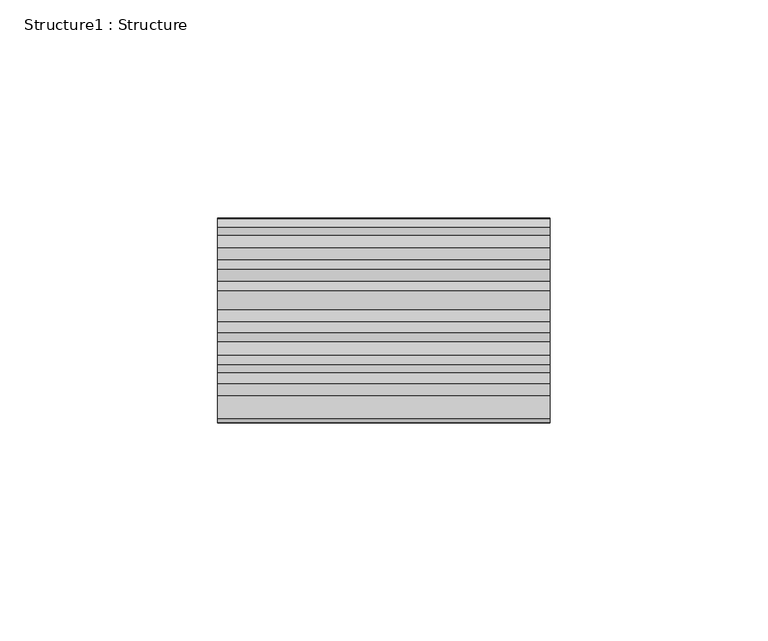
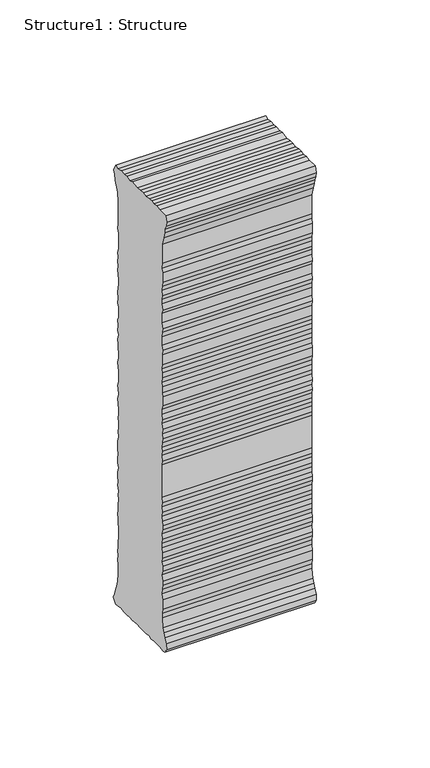
"""IFC4 building model written with IfcOpenShell, lengths in millimetres: proxy geometry, Structure1 : Structure."""

from ifc_helpers import new_model, si_unit, frame, origin, place, context, project, spatial, polyline, outline, extrude, source, transform, mapped, element, save


def structure1_structure_dc86aa21(model_context):
    return source(origin(), model_context, "Body", "SweptSolid", [
        extrude(outline(polyline([(4.3408461, 0.0), (7.4915501, 0.7019795), (10.0554785, 1.7641265), (12.8684065, 2.182644), (15.4221344, 3.2446663), (17.7447891, 0.9097053), (17.5914422, -1.249402), (16.7701535, -3.9878638), (17.2621815, -5.8853558), (17.0652013, -8.6588156), (16.583314, -11.10289), (16.7367209, -13.2837839), (16.2544134, -15.7337736), (15.783812, -17.8754442), (15.925873, -20.3595869), (15.5309522, -25.9200273), (15.0391643, -28.3600013), (15.5312523, -30.2566482), (14.7102638, -32.9908849), (14.895538, -34.8665902), (14.676471, -37.951029), (14.8080312, -40.4395218), (14.3697172, -42.2700885), (12.0906958, -43.6616211), (9.0365541, -43.1355555), (6.6577749, -41.7223611), (4.5551523, -40.6421773), (2.4618252, -39.5626537), (-2.4237884, -38.5990591), (-4.8896493, -38.4239256), (-7.3870776, -38.5497553), (-12.3154193, -38.1997283), (-15.0692673, -37.3917852), (-17.8603486, -37.5027039), (-20.0408824, -37.6510405), (-22.1999896, -37.4976936), (-25.2428454, -36.6692243), (-27.7528246, -37.103313), (-30.2279812, -36.9275193), (-32.3302944, -36.1658504), (-34.5256142, -36.3190821), (-37.2948487, -36.1224019), (-39.7397081, -35.6396095), (-42.2148647, -35.4638157), (-44.6991921, -35.5965211), (-47.4508053, -35.0919421), (-49.9700801, -35.5253706), (-52.1291874, -35.3720237), (-54.2668681, -34.9169934), (-56.7075021, -34.4345011), (-59.1960548, -34.5669064), (-61.9662591, -34.0610069), (-64.1379175, -34.2159191), (-66.8988262, -33.7106798), (-84.4911136, -32.4612178), (-86.3644685, -32.6373164), (-89.4329761, -32.1102305), (-91.9164586, -32.2429959), (-93.7520356, -31.8034767), (-96.5431169, -31.9143954), (-98.7236506, -32.062732), (-101.1782258, -31.5851947), (-103.9688869, -31.6901981), (-106.6990734, -30.8839355), (-108.8893229, -31.0375273), (-111.6367108, -30.5332483), (-114.1118673, -30.3574546), (-116.6218467, -30.7915433), (-121.2569554, -30.4623427), (-123.3861856, -30.0079125), (-126.4714696, -29.7887855), (-128.6095752, -29.3277798), (-131.4141773, -29.4377382), (-133.876658, -29.2628447), (-136.0139186, -28.801899), (-138.1940275, -28.956211), (-143.7612283, -28.5608101), (-146.23415, -28.6883803), (-148.6677234, -27.9031842), (-152.9994586, -27.5955302), (-155.7913851, -27.7063889), (-157.9583979, -27.8556858), (-160.7114009, -27.0478027), (-165.6397427, -26.6977757), (-167.8429683, -27.1536511), (-170.884979, -26.3252418), (-173.3508399, -26.1501083), (-175.2250401, -26.3261469), (-177.973273, -25.8218079), (-180.4753465, -25.9532529), (-182.6558803, -26.1015895), (-187.9002715, -25.7291156), (-190.0161054, -24.9664864), (-192.8207075, -25.0764448), (-202.9942856, -24.3538839), (-207.4152177, -25.2781952), (-210.5567461, -25.9825249), (-212.7480806, -26.1394369), (-214.9636724, -26.912927), (-217.4693015, -27.3575164), (-220.5031113, -26.2103473), (-220.1306374, -20.9659562), (-220.2409559, -18.1664244), (-219.7578034, -15.7164947), (-219.933842, -13.8422946), (-219.7804351, -11.6823424), (-218.9511807, -8.6403917), (-219.4079012, -6.4371061), (-218.9251688, -3.9930919), (-218.4256601, -1.2411185), (-218.7287336, 3.1254994), (-217.9651993, 5.2421184), (-218.3780464, 8.0631368), (-217.9167405, 10.2054676), (-218.0273592, 13.0007741), (-217.2198914, 15.735971), (-217.6984586, 17.6316577), (-214.1595897, 19.2428622), (-212.3826721, 18.1807151), (-209.3192348, 17.6539894), (-204.5660866, 14.8372562), (-199.6451656, 14.1794551), (-187.9226078, 13.3468806), (-185.1172206, 13.4559339), (-183.0028919, 12.6840692), (-174.9749002, 12.1138949), (-172.4634157, 12.5572192), (-170.0244117, 12.0756919), (-167.8426728, 12.2290388), (-165.0817041, 11.7246446), (-162.8999651, 11.8779915), (-160.4550457, 11.3960441), (-158.3172402, 10.9308132), (-155.8420836, 10.7550195), (-150.8698084, 11.0235703), (-148.1088397, 10.5191761), (-145.3169734, 10.6291897), (-143.1891238, 9.8563647), (-137.9574085, 9.4847911), (-136.0568964, 9.9715086), (-132.9933991, 9.4456278), (-130.5040613, 9.577128), (-128.380437, 8.8046032), (-125.8697976, 9.2479874), (-123.1223496, 8.7445535), (-120.9632424, 8.5912066), (-118.517838, 8.104129), (-116.0426815, 7.9283353), (-113.2159927, 8.3492727), (-108.9408666, 7.4239411), (-103.3888766, 7.0296205), (-100.8833074, 7.4733649), (-99.0476703, 7.0346907), (-96.5938155, 6.5470129), (-94.0882464, 6.9907573), (-91.0340446, 6.4655367), (-88.5801898, 5.9778589), (-86.1134837, 5.8026654), (-83.6246309, 5.9392958), (-81.1716211, 5.4516781), (-78.7091403, 5.2767846), (-76.211837, 5.4128149), (-73.7672777, 4.9257973), (-71.2566383, 5.3691815), (-66.9375787, 5.0624278), (-64.1808352, 4.5583336), (-61.9999414, 4.7117405), (-59.2264815, 4.5147603), (-57.1020122, 3.7421754), (-54.2888442, 4.1640731), (-51.8221381, 3.9888795), (-49.6704517, 3.5277586), (-47.1870292, 3.6596789), (-44.4482073, 2.8434607), (-42.2661083, 3.0018778), (-39.8215489, 2.5148602), (-37.3377665, 2.6518508), (-34.2524826, 2.4327238), (-32.0707436, 2.5860707), (-29.6123034, 2.103163), (-26.8430688, 1.9064829), (-25.0137072, 1.4631587), (-19.4608722, 1.0687781), (-17.5821467, 1.2487418), (-14.4968628, 1.0296148), (-12.0083701, 1.161175), (-9.5541551, 0.6785675), (-7.6893106, 0.8544212), (-4.6258134, 0.3285405), (0.0, 0.0), (4.3408461, 0.0)])), frame((-35624.0862846, 275042.9553921, 4000.1487179), z_axis=(1.0, 0.0, 1.3542500454377657e-12), x_axis=(1.3521812008529227e-12, 0.07084482636111814, -0.9974873485803533)), (0.0, 0.0, 1.0), 76.2),
    ])


if __name__ == "__main__":
    model = new_model("IFC4")
    model_context = context("Model", 3, world=origin())
    ifc_project = project(units=[si_unit("LENGTHUNIT", "METRE", prefix="MILLI")], contexts=[model_context])
    site = spatial("IfcSite", under=ifc_project)
    building = spatial("IfcBuilding", under=site)
    placement = place(None, origin())
    structure1_structure_shape = structure1_structure_dc86aa21(model_context)
    element("IfcBuildingElementProxy", 1, Name="Structure1 : Structure", ObjectType="Structure1 : Structure", at=placement, inside=building, context=model_context, shape_type="MappedRepresentation", body=[
        mapped(structure1_structure_shape, transform((0.0, 0.0, 0.0), x_axis=(1.0, 0.0, 0.0), y_axis=(0.0, 1.0, 0.0), z_axis=(0.0, 0.0, 1.0))),
    ])
    save(model, "model.ifc")

# Revit data of these elements
# Type "Structure1 : Structure"
#   NameOverride = "Structure"
# Element 1 (IfcBuildingElementProxy, "Structure1 : Structure")
#   Materials on its faces: "BRUSHED ALUMINUM LETTERING"
# Materials
#   "BRUSHED ALUMINUM LETTERING": class "Unassigned", colour RGB 169 181 186, transparency 0, Cost = 0
